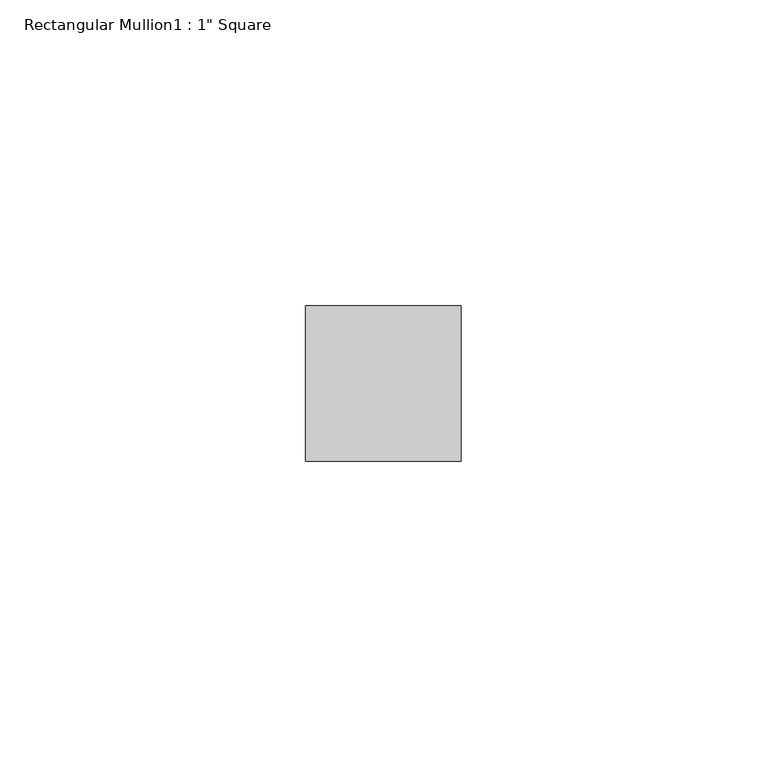
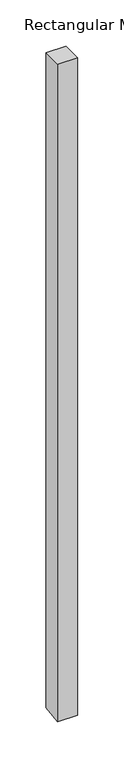
"""IFC4 building model written with IfcOpenShell, lengths in millimetres: member geometry."""

import ifcopenshell
import ifcopenshell.guid

model = None  # the IFC model being written
_history = None  # IfcOwnerHistory: only IFC2X3 demands one
_inside = {}  # id of a spatial element -> (the spatial element, [elements in it])
_under = {}  # id of a project, library or spatial element -> (it, [spatial elements below it])
_declared = {}  # id of a project -> (the project, [libraries it declares])
_typed = {}  # id of a type object -> (the type object, [elements of that type])
_made_of = {}  # id of a material, layer set ... -> (it, [elements and type objects made of it])


def new_model(schema):
    """Start an empty IFC model of exactly this schema.

    Asked for "IFC4X3", IfcOpenShell would pick the latest addendum, in which some entities
    have other attributes; the version numbers below select the first issue.
    IFC2X3 requires an IfcOwnerHistory on every rooted entity: one is made here for all.
    """
    global model, _history
    if schema == "IFC4X3":
        model = ifcopenshell.file(schema_version=(4, 3, 0, 0))
    else:
        model = ifcopenshell.file(schema=schema)
    _inside.clear()
    _under.clear()
    _declared.clear()
    _typed.clear()
    _made_of.clear()
    _history = None
    if model.schema == "IFC2X3":
        org = make("IfcOrganization", Name="unknown")
        user = make(
            "IfcPersonAndOrganization",
            ThePerson=make("IfcPerson", FamilyName="unknown"),
            TheOrganization=org,
        )
        app = make(
            "IfcApplication",
            ApplicationDeveloper=org,
            Version="unknown",
            ApplicationFullName="unknown",
            ApplicationIdentifier="unknown",
        )
        _history = make(
            "IfcOwnerHistory",
            OwningUser=user,
            OwningApplication=app,
            ChangeAction="ADDED",
            CreationDate=0,
        )
    return model


def make(cls, **values):
    """One entity of the class cls with the attributes given. An attribute that is None is left unset."""
    return model.create_entity(
        cls, **{name: value for name, value in values.items() if value is not None}
    )


def rooted(cls, **values):
    """An entity with a GlobalId (a new one), such as an element, a storey or a relation."""
    return make(cls, GlobalId=ifcopenshell.guid.new(), OwnerHistory=_history, **values)


def si_unit(unit_type, name, prefix=None):
    """IfcSIUnit, for example si_unit("LENGTHUNIT", "METRE", prefix="MILLI")."""
    return make("IfcSIUnit", UnitType=unit_type, Prefix=prefix, Name=name)


def assignment(units):
    """IfcUnitAssignment: the units of a project."""
    return None if units is None else make("IfcUnitAssignment", Units=units)


def point(xyz):
    """IfcCartesianPoint."""
    return None if xyz is None else make("IfcCartesianPoint", Coordinates=xyz)


def direction(xyz):
    """IfcDirection."""
    return None if xyz is None else make("IfcDirection", DirectionRatios=xyz)


def frame(location, z_axis=None, x_axis=None):
    """IfcAxis2Placement3D, a coordinate frame: its origin and axes. An axis left out is left unset."""
    return make(
        "IfcAxis2Placement3D",
        Location=point(location),
        Axis=direction(z_axis),
        RefDirection=direction(x_axis),
    )


def origin():
    """The frame at (0, 0, 0) with its axes left unset."""
    return frame((0.0, 0.0, 0.0))


def place(relative_to, where):
    """IfcLocalPlacement: puts the frame where relative to a parent placement (None: the world)."""
    return make(
        "IfcLocalPlacement", PlacementRelTo=relative_to, RelativePlacement=where
    )


def context(
    kind, dimensions, precision=None, world=None, true_north=None, identifier=None
):
    """IfcGeometricRepresentationContext, for example the 3D "Model" context."""
    return make(
        "IfcGeometricRepresentationContext",
        ContextIdentifier=identifier,
        ContextType=kind,
        CoordinateSpaceDimension=dimensions,
        Precision=precision,
        WorldCoordinateSystem=world,
        TrueNorth=true_north,
    )


def project(units=None, contexts=None):
    """IfcProject with its units and contexts."""
    return rooted(
        "IfcProject",
        Name="project",
        RepresentationContexts=contexts,
        UnitsInContext=assignment(units),
    )


def spatial(cls, under=None, at=None, **own):
    """A site, building, storey or space (cls), placed at a placement, below another one or the project."""
    s = rooted(cls, ObjectPlacement=at, **own)
    if under is not None:
        _under.setdefault(under.id(), (under, []))[1].append(s)
    return s


def polyline(points):
    """IfcPolyline through the points."""
    return make("IfcPolyline", Points=[point(p) for p in points])


def outline(outer, holes=None, kind="AREA"):
    """IfcArbitraryClosedProfileDef: a profile drawn as a closed curve; with holes, ...WithVoids."""
    if holes is None:
        return make("IfcArbitraryClosedProfileDef", ProfileType=kind, OuterCurve=outer)
    return make(
        "IfcArbitraryProfileDefWithVoids",
        ProfileType=kind,
        OuterCurve=outer,
        InnerCurves=holes,
    )


def extrude(swept, where, along, depth):
    """IfcExtrudedAreaSolid: the profile swept, set in the frame where, extruded along a direction by depth."""
    return make(
        "IfcExtrudedAreaSolid",
        SweptArea=swept,
        Position=where,
        ExtrudedDirection=direction(along),
        Depth=depth,
    )


def shape(context_of_items, identifier, shape_type, items):
    """IfcShapeRepresentation: the items that make up one representation, for example the "Body"."""
    return make(
        "IfcShapeRepresentation",
        ContextOfItems=context_of_items,
        RepresentationIdentifier=identifier,
        RepresentationType=shape_type,
        Items=items,
    )


def source(mapping_origin, context_of_items, identifier, shape_type, items):
    """IfcRepresentationMap: a shape defined once, which mapped items show again and again."""
    return make(
        "IfcRepresentationMap",
        MappingOrigin=mapping_origin,
        MappedRepresentation=shape(context_of_items, identifier, shape_type, items),
    )


def transform(
    local_origin,
    x_axis=None,
    y_axis=None,
    z_axis=None,
    scale=None,
    scale2=None,
    scale3=None,
    uniform=True,
):
    """IfcCartesianTransformationOperator3D, or its non-uniform kind. x_axis, y_axis, z_axis: its Axis1, 2, 3."""
    if uniform:
        return make(
            "IfcCartesianTransformationOperator3D",
            Axis1=direction(x_axis),
            Axis2=direction(y_axis),
            LocalOrigin=point(local_origin),
            Scale=scale,
            Axis3=direction(z_axis),
        )
    return make(
        "IfcCartesianTransformationOperator3DnonUniform",
        Axis1=direction(x_axis),
        Axis2=direction(y_axis),
        LocalOrigin=point(local_origin),
        Scale=scale,
        Axis3=direction(z_axis),
        Scale2=scale2,
        Scale3=scale3,
    )


def mapped(mapping_source, mapping_target):
    """IfcMappedItem: shows the shape of a source again, moved by a transform."""
    return make(
        "IfcMappedItem", MappingSource=mapping_source, MappingTarget=mapping_target
    )


def made_of(thing, what):
    """Note that an element or type object is made of a material, layer set ...; save() writes the relation."""
    if what is not None:
        _made_of.setdefault(what.id(), (what, []))[1].append(thing)
    return thing


def element(
    cls,
    number,
    at=None,
    inside=None,
    cuts=None,
    type_object=None,
    material=None,
    context=None,
    identifier="Body",
    shape_type=None,
    held_by="IfcProductDefinitionShape",
    body=None,
    shapes=None,
    **own,
):
    """One element of the class cls, such as IfcWall. Its Tag is "e" and its number.

    at: its placement. inside: the storey or other place that contains it. cuts: it is an
    opening in that element (IfcRelVoidsElement). A single representation is given by context,
    identifier, shape_type and body (its items); several are given by shapes. held_by: the class
    of the entity that holds the representations. save() writes the other relations.
    """
    e = rooted(cls, Tag="e%d" % number, ObjectPlacement=at, **own)
    if body is not None:
        shapes = [shape(context, identifier, shape_type, body)]
    if shapes is not None:
        e.Representation = make(held_by, Representations=shapes)
    if inside is not None:
        _inside.setdefault(inside.id(), (inside, []))[1].append(e)
    if cuts is not None:
        rooted(
            "IfcRelVoidsElement", RelatingBuildingElement=cuts, RelatedOpeningElement=e
        )
    if type_object is not None:
        _typed.setdefault(type_object.id(), (type_object, []))[1].append(e)
    return made_of(e, material)


def aggregate(whole, parts):
    """IfcRelAggregates: a whole, such as a stair, and the parts it consists of."""
    return rooted("IfcRelAggregates", RelatingObject=whole, RelatedObjects=parts)


def save(model, path):
    """Write the relations noted so far, then the file.

    IfcRelAggregates (storeys below a building ...), IfcRelContainedInSpatialStructure (elements
    in a storey), IfcRelDefinesByType, IfcRelAssociatesMaterial and IfcRelDeclares: one each for
    every whole, place, type object, material and project.
    """
    for whole, parts in _under.values():
        aggregate(whole, parts)
    for where, things in _inside.values():
        rooted(
            "IfcRelContainedInSpatialStructure",
            RelatedElements=things,
            RelatingStructure=where,
        )
    for kind, things in _typed.values():
        rooted("IfcRelDefinesByType", RelatedObjects=things, RelatingType=kind)
    for what, things in _made_of.values():
        rooted("IfcRelAssociatesMaterial", RelatedObjects=things, RelatingMaterial=what)
    for by, libraries in _declared.values():
        rooted("IfcRelDeclares", RelatingContext=by, RelatedDefinitions=libraries)
    model.write(path)


def member_834e91f0(model_context):
    return source(origin(), model_context, "Body", "SweptSolid", [
        extrude(outline(polyline([(-44.45, 0.0), (-19.05, 0.0), (-19.05, -868.6621003), (-44.45, -871.9742504), (-44.45, 0.0)])), frame((-25.4, 0.0, 0.0), z_axis=(1.0, 0.0, 0.0), x_axis=(0.0, 1.0, 0.0)), (0.0, 0.0, 1.0), 25.4),
    ])


if __name__ == "__main__":
    model = new_model("IFC4")
    model_context = context("Model", 3, world=origin())
    ifc_project = project(units=[si_unit("LENGTHUNIT", "METRE", prefix="MILLI")], contexts=[model_context])
    site = spatial("IfcSite", under=ifc_project)
    building = spatial("IfcBuilding", under=site)
    placement = place(None, origin())
    member_shape = member_834e91f0(model_context)
    element("IfcMember", 1, ObjectType="Rectangular Mullion1 : 1\" Square", at=placement, inside=building, context=model_context, shape_type="MappedRepresentation", body=[
        mapped(member_shape, transform((0.0, 0.0, 0.0), x_axis=(1.0, 0.0, 0.0), y_axis=(0.0, 1.0, 0.0), z_axis=(0.0, 0.0, 1.0))),
    ])
    save(model, "model.ifc")

# Revit data of these elements
# Type "Rectangular Mullion1 : 1\" Square"
#   built-in parameter 1007351 = 0.104167 (stored number, unit not read)
#   built-in parameter 1007304 = 0.0833333 (stored number, unit not read)
#   built-in parameter 1007301 = 0.0416667 (stored number, unit not read)
#   built-in parameter 1007300 = 0.0416667 (stored number, unit not read)
